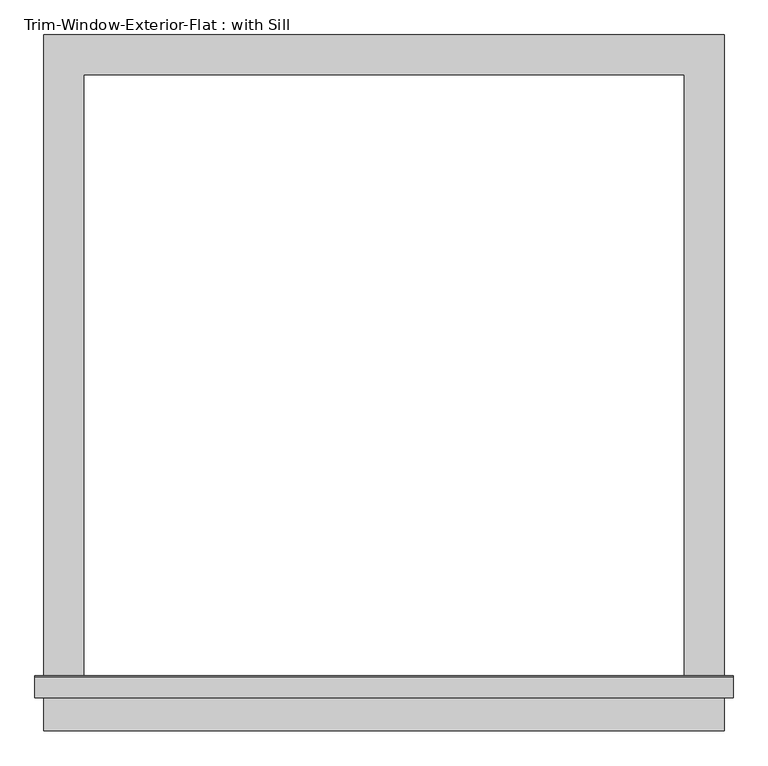
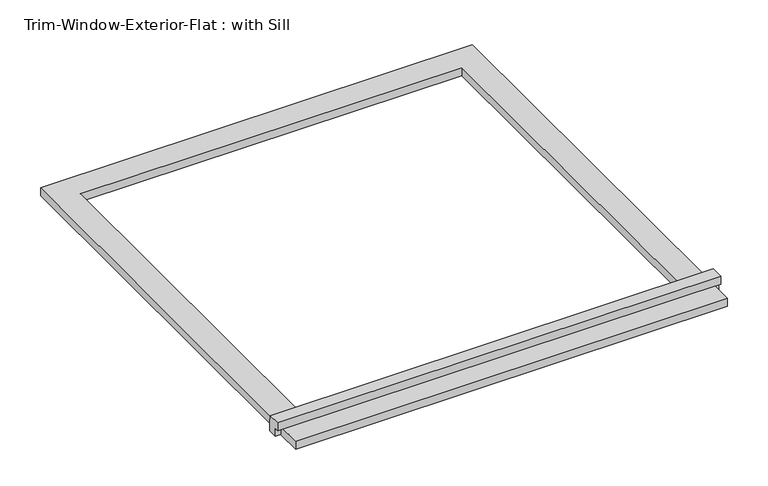
"""IFC4 building model written with IfcOpenShell, lengths in millimetres: proxy geometry, Trim-Window-Exterior-Flat : with Sill."""

import ifcopenshell
import ifcopenshell.guid

model = None  # the IFC model being written
_history = None  # IfcOwnerHistory: only IFC2X3 demands one
_inside = {}  # id of a spatial element -> (the spatial element, [elements in it])
_under = {}  # id of a project, library or spatial element -> (it, [spatial elements below it])
_declared = {}  # id of a project -> (the project, [libraries it declares])
_typed = {}  # id of a type object -> (the type object, [elements of that type])
_made_of = {}  # id of a material, layer set ... -> (it, [elements and type objects made of it])


def new_model(schema):
    """Start an empty IFC model of exactly this schema.

    Asked for "IFC4X3", IfcOpenShell would pick the latest addendum, in which some entities
    have other attributes; the version numbers below select the first issue.
    IFC2X3 requires an IfcOwnerHistory on every rooted entity: one is made here for all.
    """
    global model, _history
    if schema == "IFC4X3":
        model = ifcopenshell.file(schema_version=(4, 3, 0, 0))
    else:
        model = ifcopenshell.file(schema=schema)
    _inside.clear()
    _under.clear()
    _declared.clear()
    _typed.clear()
    _made_of.clear()
    _history = None
    if model.schema == "IFC2X3":
        org = make("IfcOrganization", Name="unknown")
        user = make(
            "IfcPersonAndOrganization",
            ThePerson=make("IfcPerson", FamilyName="unknown"),
            TheOrganization=org,
        )
        app = make(
            "IfcApplication",
            ApplicationDeveloper=org,
            Version="unknown",
            ApplicationFullName="unknown",
            ApplicationIdentifier="unknown",
        )
        _history = make(
            "IfcOwnerHistory",
            OwningUser=user,
            OwningApplication=app,
            ChangeAction="ADDED",
            CreationDate=0,
        )
    return model


def make(cls, **values):
    """One entity of the class cls with the attributes given. An attribute that is None is left unset."""
    return model.create_entity(
        cls, **{name: value for name, value in values.items() if value is not None}
    )


def rooted(cls, **values):
    """An entity with a GlobalId (a new one), such as an element, a storey or a relation."""
    return make(cls, GlobalId=ifcopenshell.guid.new(), OwnerHistory=_history, **values)


def si_unit(unit_type, name, prefix=None):
    """IfcSIUnit, for example si_unit("LENGTHUNIT", "METRE", prefix="MILLI")."""
    return make("IfcSIUnit", UnitType=unit_type, Prefix=prefix, Name=name)


def assignment(units):
    """IfcUnitAssignment: the units of a project."""
    return None if units is None else make("IfcUnitAssignment", Units=units)


def point(xyz):
    """IfcCartesianPoint."""
    return None if xyz is None else make("IfcCartesianPoint", Coordinates=xyz)


def direction(xyz):
    """IfcDirection."""
    return None if xyz is None else make("IfcDirection", DirectionRatios=xyz)


def frame(location, z_axis=None, x_axis=None):
    """IfcAxis2Placement3D, a coordinate frame: its origin and axes. An axis left out is left unset."""
    return make(
        "IfcAxis2Placement3D",
        Location=point(location),
        Axis=direction(z_axis),
        RefDirection=direction(x_axis),
    )


def origin():
    """The frame at (0, 0, 0) with its axes left unset."""
    return frame((0.0, 0.0, 0.0))


def origin_with_axes():
    """The frame at (0, 0, 0) with the z axis (0, 0, 1) and the x axis (1, 0, 0) written out."""
    return frame((0.0, 0.0, 0.0), z_axis=(0.0, 0.0, 1.0), x_axis=(1.0, 0.0, 0.0))


def place(relative_to, where):
    """IfcLocalPlacement: puts the frame where relative to a parent placement (None: the world)."""
    return make(
        "IfcLocalPlacement", PlacementRelTo=relative_to, RelativePlacement=where
    )


def context(
    kind, dimensions, precision=None, world=None, true_north=None, identifier=None
):
    """IfcGeometricRepresentationContext, for example the 3D "Model" context."""
    return make(
        "IfcGeometricRepresentationContext",
        ContextIdentifier=identifier,
        ContextType=kind,
        CoordinateSpaceDimension=dimensions,
        Precision=precision,
        WorldCoordinateSystem=world,
        TrueNorth=true_north,
    )


def project(units=None, contexts=None):
    """IfcProject with its units and contexts."""
    return rooted(
        "IfcProject",
        Name="project",
        RepresentationContexts=contexts,
        UnitsInContext=assignment(units),
    )


def spatial(cls, under=None, at=None, **own):
    """A site, building, storey or space (cls), placed at a placement, below another one or the project."""
    s = rooted(cls, ObjectPlacement=at, **own)
    if under is not None:
        _under.setdefault(under.id(), (under, []))[1].append(s)
    return s


def polyline(points):
    """IfcPolyline through the points."""
    return make("IfcPolyline", Points=[point(p) for p in points])


def outline(outer, holes=None, kind="AREA"):
    """IfcArbitraryClosedProfileDef: a profile drawn as a closed curve; with holes, ...WithVoids."""
    if holes is None:
        return make("IfcArbitraryClosedProfileDef", ProfileType=kind, OuterCurve=outer)
    return make(
        "IfcArbitraryProfileDefWithVoids",
        ProfileType=kind,
        OuterCurve=outer,
        InnerCurves=holes,
    )


def extrude(swept, where, along, depth):
    """IfcExtrudedAreaSolid: the profile swept, set in the frame where, extruded along a direction by depth."""
    return make(
        "IfcExtrudedAreaSolid",
        SweptArea=swept,
        Position=where,
        ExtrudedDirection=direction(along),
        Depth=depth,
    )


def shape(context_of_items, identifier, shape_type, items):
    """IfcShapeRepresentation: the items that make up one representation, for example the "Body"."""
    return make(
        "IfcShapeRepresentation",
        ContextOfItems=context_of_items,
        RepresentationIdentifier=identifier,
        RepresentationType=shape_type,
        Items=items,
    )


def source(mapping_origin, context_of_items, identifier, shape_type, items):
    """IfcRepresentationMap: a shape defined once, which mapped items show again and again."""
    return make(
        "IfcRepresentationMap",
        MappingOrigin=mapping_origin,
        MappedRepresentation=shape(context_of_items, identifier, shape_type, items),
    )


def transform(
    local_origin,
    x_axis=None,
    y_axis=None,
    z_axis=None,
    scale=None,
    scale2=None,
    scale3=None,
    uniform=True,
):
    """IfcCartesianTransformationOperator3D, or its non-uniform kind. x_axis, y_axis, z_axis: its Axis1, 2, 3."""
    if uniform:
        return make(
            "IfcCartesianTransformationOperator3D",
            Axis1=direction(x_axis),
            Axis2=direction(y_axis),
            LocalOrigin=point(local_origin),
            Scale=scale,
            Axis3=direction(z_axis),
        )
    return make(
        "IfcCartesianTransformationOperator3DnonUniform",
        Axis1=direction(x_axis),
        Axis2=direction(y_axis),
        LocalOrigin=point(local_origin),
        Scale=scale,
        Axis3=direction(z_axis),
        Scale2=scale2,
        Scale3=scale3,
    )


def mapped(mapping_source, mapping_target):
    """IfcMappedItem: shows the shape of a source again, moved by a transform."""
    return make(
        "IfcMappedItem", MappingSource=mapping_source, MappingTarget=mapping_target
    )


def made_of(thing, what):
    """Note that an element or type object is made of a material, layer set ...; save() writes the relation."""
    if what is not None:
        _made_of.setdefault(what.id(), (what, []))[1].append(thing)
    return thing


def element(
    cls,
    number,
    at=None,
    inside=None,
    cuts=None,
    type_object=None,
    material=None,
    context=None,
    identifier="Body",
    shape_type=None,
    held_by="IfcProductDefinitionShape",
    body=None,
    shapes=None,
    **own,
):
    """One element of the class cls, such as IfcWall. Its Tag is "e" and its number.

    at: its placement. inside: the storey or other place that contains it. cuts: it is an
    opening in that element (IfcRelVoidsElement). A single representation is given by context,
    identifier, shape_type and body (its items); several are given by shapes. held_by: the class
    of the entity that holds the representations. save() writes the other relations.
    """
    e = rooted(cls, Tag="e%d" % number, ObjectPlacement=at, **own)
    if body is not None:
        shapes = [shape(context, identifier, shape_type, body)]
    if shapes is not None:
        e.Representation = make(held_by, Representations=shapes)
    if inside is not None:
        _inside.setdefault(inside.id(), (inside, []))[1].append(e)
    if cuts is not None:
        rooted(
            "IfcRelVoidsElement", RelatingBuildingElement=cuts, RelatedOpeningElement=e
        )
    if type_object is not None:
        _typed.setdefault(type_object.id(), (type_object, []))[1].append(e)
    return made_of(e, material)


def aggregate(whole, parts):
    """IfcRelAggregates: a whole, such as a stair, and the parts it consists of."""
    return rooted("IfcRelAggregates", RelatingObject=whole, RelatedObjects=parts)


def save(model, path):
    """Write the relations noted so far, then the file.

    IfcRelAggregates (storeys below a building ...), IfcRelContainedInSpatialStructure (elements
    in a storey), IfcRelDefinesByType, IfcRelAssociatesMaterial and IfcRelDeclares: one each for
    every whole, place, type object, material and project.
    """
    for whole, parts in _under.values():
        aggregate(whole, parts)
    for where, things in _inside.values():
        rooted(
            "IfcRelContainedInSpatialStructure",
            RelatedElements=things,
            RelatingStructure=where,
        )
    for kind, things in _typed.values():
        rooted("IfcRelDefinesByType", RelatedObjects=things, RelatingType=kind)
    for what, things in _made_of.values():
        rooted("IfcRelAssociatesMaterial", RelatedObjects=things, RelatingMaterial=what)
    for by, libraries in _declared.values():
        rooted("IfcRelDeclares", RelatingContext=by, RelatedDefinitions=libraries)
    model.write(path)


def trim_window_exterior_flat_with_sill_a8480fd4(model_context):
    return source(origin(), model_context, "Body", "SweptSolid", [
        extrude(outline(polyline([(488.95, -885.7823709), (488.95, -942.9323709), (-488.95, -942.9323709), (-488.95, -885.7823709), (488.95, -885.7823709)])), origin_with_axes(), (0.0, 0.0, 1.0), 19.05),
        extrude(outline(polyline([(-895.35, 38.1), (-866.0580645, 38.1), (-863.6, 19.05), (-863.6, 0.0), (-885.7823709, 0.0), (-885.7823709, 19.05), (-895.35, 19.05), (-895.35, 38.1)])), frame((-501.65, 0.0, 0.0), z_axis=(1.0, 0.0, 0.0), x_axis=(0.0, 1.0, 0.0)), (0.0, 0.0, 1.0), 1003.3),
        extrude(outline(polyline([(-488.95, 57.15), (488.95, 57.15), (488.95, -863.6), (431.8, -863.6), (431.8, 0.0), (-431.8, 0.0), (-431.8, -863.6), (-488.95, -863.6), (-488.95, 57.15)])), origin_with_axes(), (0.0, 0.0, 1.0), 19.05),
    ])


if __name__ == "__main__":
    model = new_model("IFC4")
    model_context = context("Model", 3, world=origin())
    ifc_project = project(units=[si_unit("LENGTHUNIT", "METRE", prefix="MILLI")], contexts=[model_context])
    site = spatial("IfcSite", under=ifc_project)
    building = spatial("IfcBuilding", under=site)
    placement = place(None, origin())
    trim_window_exterior_flat_with_sill_shape = trim_window_exterior_flat_with_sill_a8480fd4(model_context)
    element("IfcBuildingElementProxy", 1, Name="Trim-Window-Exterior-Flat : with Sill", ObjectType="Trim-Window-Exterior-Flat : with Sill", at=placement, inside=building, context=model_context, shape_type="MappedRepresentation", body=[
        mapped(trim_window_exterior_flat_with_sill_shape, transform((0.0, 0.0, 0.0), x_axis=(1.0, 0.0, 0.0), y_axis=(0.0, 1.0, 0.0), z_axis=(0.0, 0.0, 1.0))),
    ])
    save(model, "model.ifc")

# Revit data of these elements
# Type "Trim-Window-Exterior-Flat : with Sill"
#   Trim Width = 0' - 2 1/4"
#   Trim Thickness_Picture Frame = 0' - 1 1/4"
#   Trim Thickness_with Sill = 0' - 0 3/4"
#   Sill Thickness = 0' - 1 1/4"
#   Opening Width [instance default] = 2' - 0"
#   Opening Height [instance default] = 3' - 0"
#   Default Elevation = 4' - 0"
#   Sill = yes
#   Picture Frame = no
#   Trim Material [instance default] = none
# Element 1 (IfcBuildingElementProxy, "Trim-Window-Exterior-Flat : with Sill")
#   Opening Width = 2' - 10"
#   Opening Height = 2' - 10"
#   Trim Material = Clad - White
#   Materials on its faces: "Clad - White"
# Materials
#   "Clad - White": class "Wood", colour RGB 242 242 238, transparency 0, Cost = 0
